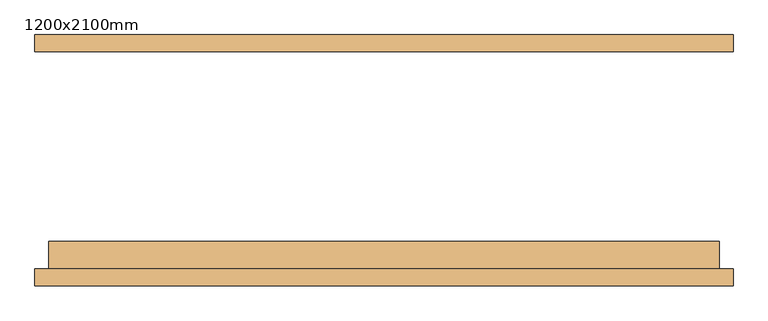
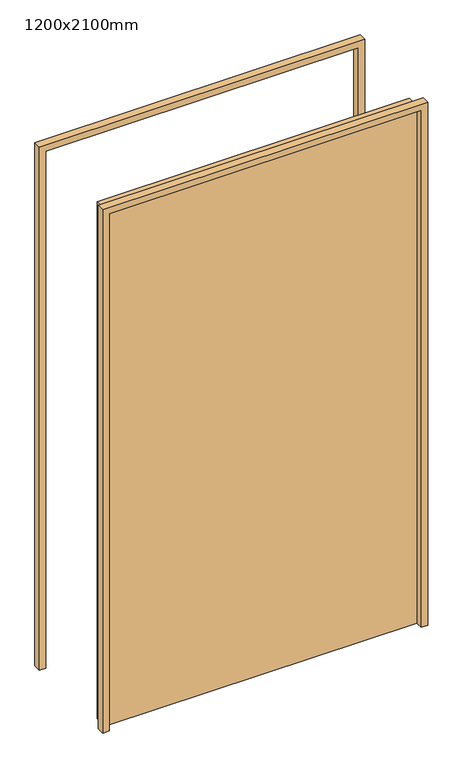
"""IFC4 building model written with IfcOpenShell, lengths in millimetres: door geometry, WWm-SingleSolid-Flush : 1200x2100mm."""

from ifc_helpers import new_model, si_unit, frame, origin, origin_with_axes, place, context, project, spatial, polyline, outline, extrude, source, transform, mapped, element, save


def door_1200x2100mm_7cba0f5e(model_context):
    return source(origin(), model_context, "Body", "SweptSolid", [
        extrude(outline(polyline([(2125.0, -625.0), (0.0, -625.0), (0.0, -600.0), (2100.0, -600.0), (2100.0, 600.0), (0.0, 600.0), (0.0, 625.0), (2125.0, 625.0), (2125.0, -625.0)])), frame((0.0, -225.0, 0.0), z_axis=(0.0, 1.0, 0.0), x_axis=(0.0, 0.0, 1.0)), (0.0, 0.0, 1.0), 30.0),
        extrude(outline(polyline([(2125.0, 625.0), (2125.0, -625.0), (0.0, -625.0), (0.0, -600.0), (2100.0, -600.0), (2100.0, 600.0), (0.0, 600.0), (0.0, 625.0), (2125.0, 625.0)])), frame((0.0, 195.0, 0.0), z_axis=(0.0, 1.0, 0.0), x_axis=(0.0, 0.0, 1.0)), (0.0, 0.0, 1.0), 30.0),
        extrude(outline(polyline([(600.0, -145.0), (600.0, -195.0), (-600.0, -195.0), (-600.0, -145.0), (600.0, -145.0)])), origin_with_axes(), (0.0, 0.0, 1.0), 2100.0),
    ])


if __name__ == "__main__":
    model = new_model("IFC4")
    model_context = context("Model", 3, world=origin())
    ifc_project = project(units=[si_unit("LENGTHUNIT", "METRE", prefix="MILLI")], contexts=[model_context])
    site = spatial("IfcSite", under=ifc_project)
    building = spatial("IfcBuilding", under=site)
    placement = place(None, origin())
    door_1200x2100mm_shape = door_1200x2100mm_7cba0f5e(model_context)
    element("IfcDoor", 1, ObjectType="WWm-SingleSolid-Flush : 1200x2100mm", at=placement, inside=building, context=model_context, shape_type="MappedRepresentation", body=[
        mapped(door_1200x2100mm_shape, transform((0.0, 0.0, 0.0), x_axis=(1.0, 0.0, 0.0), y_axis=(0.0, 1.0, 0.0), z_axis=(0.0, 0.0, 1.0))),
    ])
    save(model, "model.ifc")

# Revit data of these elements
# Type "WWm-SingleSolid-Flush : 1200x2100mm"
#   Type Mark = "EX1-55"
#   Construction Type Id = "MDOOR"
#   Assembly Code = "C1020"
#   Analytic Construction = "Metal"
#   Thickness = 50 mm
#   Thermal Resistance (R) = 0.270117 (m²·K)/W
#   Heat Transfer Coefficient (U) = 3.7021 W/(m²·K)
#   Height = 2100 mm
#   Trim Projection Ext = 30 mm
#   Trim Projection Int = 30 mm
#   Trim Width = 25 mm
#   Width = 1200 mm
#   Not 90 Degree [instance default] = no
#   90 Degree [instance default] = yes
#   Door Material = WW-EC-RGB-White
#   Frame Material = WW-EC-RGB-White
#   Visual Light Transmittance = 0
#   Solar Heat Gain Coefficient = 0
#   Function = (empty or 0)
#   Wall Closure = (empty or 0)
# Element 1 (IfcDoor, "WWm-SingleSolid-Flush : 1200x2100mm")
#   Materials on its faces: "WW-EC-RGB-White"
# Materials
#   "WW-EC-RGB-White": class "Generic", colour RGB 255 255 255, transparency 0, Comments = "If region requests off-white, swith asset color to RGB 231-228-220", Description = "Generic Color", Cost = 0
